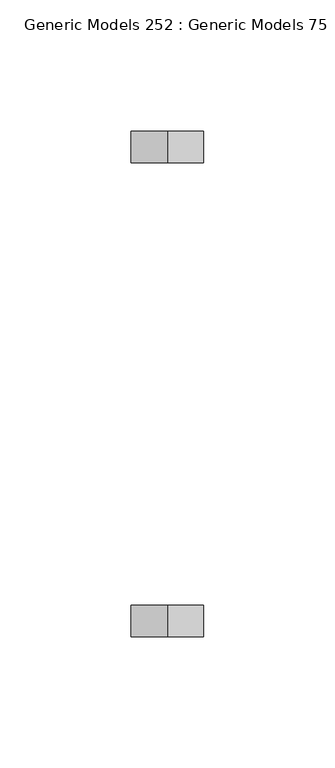
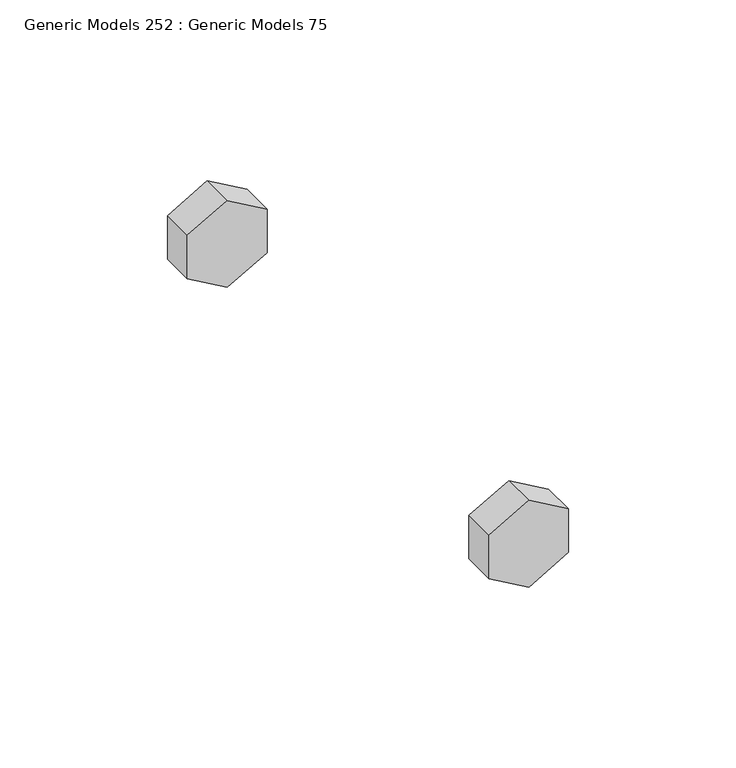
"""IFC4 building model written with IfcOpenShell, lengths in millimetres: proxy geometry, Generic Models 252 : Generic Models 75."""

from ifc_helpers import new_model, si_unit, frame, origin, place, context, project, spatial, polyline, outline, extrude, source, transform, mapped, element, save


def generic_models_252_generic_models_75_131dc0a8(model_context):
    return source(origin(), model_context, "Body", "SweptSolid", [
        extrude(outline(polyline([(269298.5462802, 31975.9942029), (269282.7097067, 31975.9942029), (269274.79142, 31989.7090778), (269282.7097067, 32003.4239528), (269298.5462802, 32003.4239528), (269306.464567, 31989.7090778), (269298.5462802, 31975.9942029)])), frame((0.0, 30858.4781612, 0.0), z_axis=(0.0, 1.0, 0.0), x_axis=(0.0, 0.0, 1.0)), (0.0, 0.0, 1.0), 11.90625),
        extrude(outline(polyline([(269298.5462802, 31975.9942029), (269282.7097067, 31975.9942029), (269274.79142, 31989.7090778), (269282.7097067, 32003.4239528), (269298.5462802, 32003.4239528), (269306.464567, 31989.7090778), (269298.5462802, 31975.9942029)])), frame((0.0, 30678.2969112, 0.0), z_axis=(0.0, 1.0, 0.0), x_axis=(0.0, 0.0, 1.0)), (0.0, 0.0, 1.0), 11.90625),
    ])


if __name__ == "__main__":
    model = new_model("IFC4")
    model_context = context("Model", 3, world=origin())
    ifc_project = project(units=[si_unit("LENGTHUNIT", "METRE", prefix="MILLI")], contexts=[model_context])
    site = spatial("IfcSite", under=ifc_project)
    building = spatial("IfcBuilding", under=site)
    placement = place(None, origin())
    generic_models_252_generic_models_75_shape = generic_models_252_generic_models_75_131dc0a8(model_context)
    element("IfcBuildingElementProxy", 1, Name="Generic Models 252 : Generic Models 75", ObjectType="Generic Models 252 : Generic Models 75", at=placement, inside=building, context=model_context, shape_type="MappedRepresentation", body=[
        mapped(generic_models_252_generic_models_75_shape, transform((0.0, 0.0, 0.0), x_axis=(1.0, 0.0, 0.0), y_axis=(0.0, 1.0, 0.0), z_axis=(0.0, 0.0, 1.0))),
    ])
    save(model, "model.ifc")

# Revit data of these elements
# Element 1 (IfcBuildingElementProxy, "Generic Models 252 : Generic Models 75")
#   Materials on its faces: "3/4\" GALV. THRU BOLTS"
# Materials
#   "3/4\" GALV. THRU BOLTS": class "Generic", colour RGB 105 69 171, transparency 0, Cost = 0
